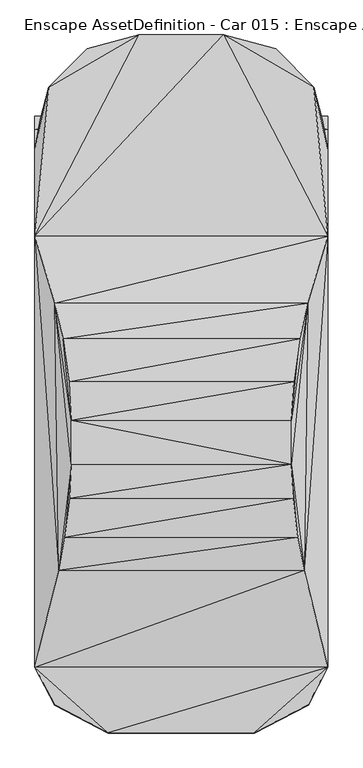
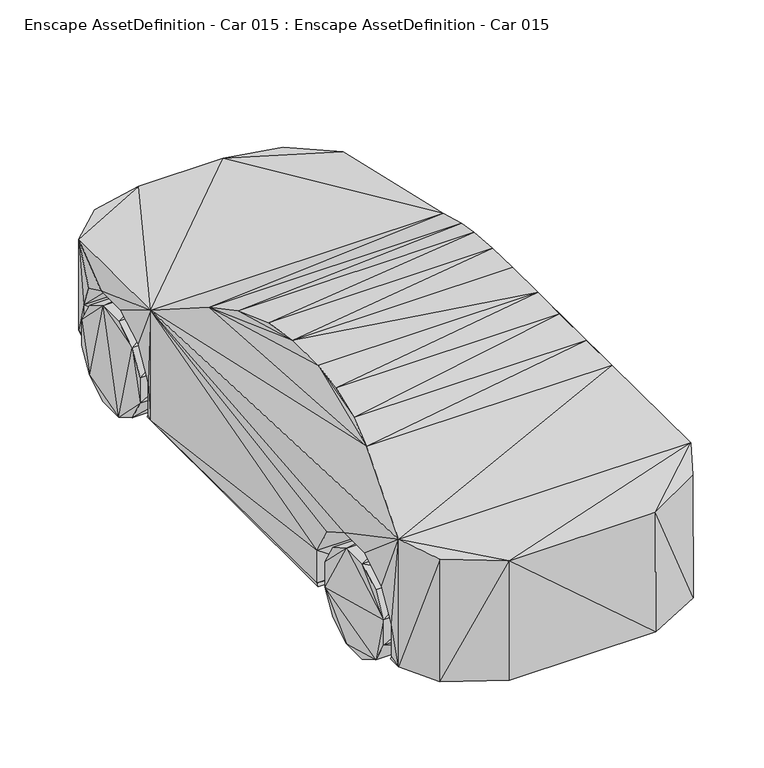
"""IFC4 building model written with IfcOpenShell, lengths in millimetres: geographic element geometry, Enscape AssetDefinition - Car 015 : Enscape AssetDefinition - Car 015."""

from ifc_helpers import new_model, si_unit, origin, place, context, project, spatial, faceted_brep, source, transform, mapped, element, save


def enscape_assetdefinition_car_015_enscape_assetdefinition_car_30b7849d(model_context):
    return source(origin(), model_context, "Body", "Brep", [
        faceted_brep([(944.226265, 1625.9566545, 237.0770574), (944.226265, 1386.8831396, 651.1646509), (944.226265, 1211.8692398, -1.9962895), (944.226265, 1538.4500027, 563.6575222), (641.0333514, 1538.4500027, 563.6575222), (641.033411, 1386.8831396, 651.1646509), (944.226265, 1211.8692398, 651.1646509), (944.226265, 1060.3027344, 563.6576414), (944.226265, 1625.9567738, 412.0909274), (944.226265, 972.7957845, 237.0771766), (641.0333514, 1625.9567738, 412.0909274), (641.0333514, 1625.9566545, 237.0770574), (641.033411, 1211.8692398, 651.1646509), (641.033411, 1060.3026152, 563.6576414), (944.226265, 972.7957845, 412.091136), (641.033411, 972.7957845, 412.091136), (641.0333514, 1211.8692398, -1.9962895), (641.0333514, 1538.449645, 85.5106041), (641.0333514, 972.7957845, 237.0771766), (944.226265, 1060.3026152, 85.5106935), (641.0333514, 1060.3026152, 85.5106935), (944.226265, 1386.8831396, -1.9963195), (944.226265, 1538.449645, 85.5105817), (641.0333514, 1386.8831396, -1.9963195)], [[[0, 1, 2]], [[3, 4, 1]], [[1, 5, 6]], [[7, 1, 6]], [[1, 0, 8]], [[1, 8, 3]], [[9, 1, 7]], [[1, 9, 2]], [[1, 4, 5]], [[10, 5, 4]], [[3, 10, 4]], [[8, 10, 3]], [[0, 11, 8]], [[8, 11, 10]], [[5, 10, 11]], [[11, 12, 5]], [[6, 5, 12]], [[6, 12, 7]], [[7, 13, 14]], [[9, 7, 14]], [[7, 12, 13]], [[15, 12, 11]], [[15, 13, 12]], [[16, 11, 17]], [[11, 16, 15]], [[0, 17, 11]], [[14, 15, 9]], [[16, 18, 15]], [[14, 13, 15]], [[9, 15, 18]], [[9, 18, 19]], [[18, 16, 20]], [[19, 18, 20]], [[19, 20, 2]], [[2, 9, 19]], [[2, 20, 16]], [[2, 16, 21]], [[22, 2, 21]], [[2, 22, 0]], [[22, 17, 0]], [[21, 23, 22]], [[22, 23, 17]], [[21, 16, 23]], [[16, 17, 23]]]),
        faceted_brep([(944.2260861, -1664.8235321, 85.5105221), (944.2260861, -1099.1698503, 237.0769083), (944.2261457, -1186.6767406, 563.657403), (944.2260861, -1186.6767406, 85.5104104), (641.0332918, -1186.6767406, 85.5104327), (944.2261457, -1099.1697311, 412.0908678), (641.0332918, -1099.1697311, 412.0908678), (944.2260861, -1338.2434845, -1.9965095), (641.0332918, -1099.1698503, 237.0769084), (641.0332918, -1338.2434845, -1.9965095), (944.2260861, -1513.2573843, -1.9964396), (641.0332918, -1513.2573843, -1.9964396), (641.0332918, -1664.8235321, 85.5105445), (641.0332918, -1186.6767406, 563.657403), (944.2261457, -1338.2434845, 651.1645317), (641.0332918, -1338.2434845, 651.1645317), (944.2261457, -1513.2570267, 651.1645317), (944.2260861, -1752.3306608, 237.0771319), (944.2260861, -1752.3306608, 412.090987), (641.0332322, -1752.3306608, 412.090987), (641.0332322, -1752.3306608, 237.0771319), (944.2261457, -1664.8238897, 563.6575818), (641.0332918, -1664.8238897, 563.6576414), (641.0332918, -1513.2570267, 651.1645317)], [[[0, 1, 2]], [[3, 4, 1]], [[5, 1, 6]], [[3, 1, 7]], [[1, 0, 7]], [[2, 1, 5]], [[1, 4, 8]], [[6, 1, 8]], [[9, 8, 4]], [[3, 9, 4]], [[7, 9, 3]], [[10, 11, 7]], [[7, 0, 10]], [[7, 11, 9]], [[11, 12, 9]], [[12, 8, 9]], [[12, 13, 8]], [[8, 13, 6]], [[2, 13, 14]], [[12, 15, 13]], [[2, 6, 13]], [[14, 13, 15]], [[14, 15, 16]], [[17, 14, 16]], [[14, 17, 0]], [[14, 0, 2]], [[5, 6, 2]], [[0, 12, 10]], [[0, 17, 12]], [[18, 19, 17]], [[18, 17, 16]], [[17, 19, 20]], [[12, 17, 20]], [[21, 22, 18]], [[18, 16, 21]], [[18, 22, 19]], [[21, 16, 22]], [[19, 22, 23]], [[22, 16, 23]], [[19, 23, 15]], [[16, 15, 23]], [[19, 15, 12]], [[19, 12, 20]], [[10, 12, 11]]]),
        faceted_brep([(-944.226265, 1060.3027344, 563.6576414), (-944.226265, 1211.8692398, -1.9962895), (-944.226265, 972.7957845, 237.0771766), (-944.226265, 1060.3026152, 85.5106935), (-641.0333514, 1060.3026152, 85.5106935), (-944.226265, 1386.8831396, -1.9963195), (-641.0333514, 1211.8692398, -1.9962895), (-944.226265, 1538.449645, 85.5105817), (-944.226265, 1386.8831396, 651.1646509), (-641.0333514, 972.7957845, 237.0771766), (-641.033411, 1386.8831396, 651.1646509), (-641.0333514, 1538.449645, 85.5106041), (-641.033411, 972.7957845, 412.091136), (-641.0333514, 1386.8831396, -1.9963195), (-944.226265, 1625.9566545, 237.0770574), (-641.0333514, 1625.9566545, 237.0770574), (-944.226265, 1625.9567738, 412.0909274), (-944.226265, 1538.4500027, 563.6575222), (-641.0333514, 1625.9567738, 412.0909274), (-641.0333514, 1538.4500027, 563.6575222), (-944.226265, 1211.8692398, 651.1646509), (-641.033411, 1211.8692398, 651.1646509), (-944.226265, 972.7957845, 412.091136), (-641.033411, 1060.3026152, 563.6576414)], [[[0, 1, 2]], [[3, 1, 4]], [[1, 5, 6]], [[1, 7, 5]], [[2, 1, 3]], [[1, 0, 8]], [[7, 1, 8]], [[4, 1, 6]], [[6, 9, 4]], [[9, 3, 4]], [[2, 3, 9]], [[10, 9, 11]], [[10, 12, 9]], [[11, 9, 6]], [[12, 2, 9]], [[11, 6, 13]], [[6, 5, 13]], [[5, 7, 13]], [[13, 7, 11]], [[7, 14, 11]], [[10, 11, 15]], [[11, 14, 15]], [[14, 16, 15]], [[7, 16, 14]], [[7, 8, 16]], [[16, 17, 18]], [[16, 8, 17]], [[15, 16, 18]], [[10, 15, 18]], [[10, 18, 19]], [[18, 17, 19]], [[17, 8, 19]], [[19, 8, 10]], [[8, 20, 10]], [[8, 0, 20]], [[20, 0, 21]], [[10, 20, 21]], [[0, 22, 23]], [[0, 2, 22]], [[21, 0, 23]], [[23, 10, 21]], [[10, 23, 12]], [[23, 22, 12]], [[22, 2, 12]]]),
        faceted_brep([(-944.2261457, -1338.2434845, 651.1645317), (-944.2260861, -1099.1698503, 237.0769083), (-944.2260861, -1752.3306608, 412.090987), (-944.2260861, -1186.6767406, 85.5104104), (-641.0332918, -1186.6767406, 85.5104327), (-641.0332918, -1099.1698503, 237.0769083), (-641.0332918, -1099.1697311, 412.0908678), (-944.2261457, -1099.1697311, 412.0908678), (-944.2260861, -1338.2434845, -1.9965095), (-944.2260861, -1664.8235321, 85.5105221), (-641.0332918, -1338.2434845, -1.9965095), (-944.2260861, -1513.2573843, -1.9964396), (-641.0332918, -1513.2573843, -1.9964396), (-641.0332918, -1664.8235321, 85.5105445), (-944.2260861, -1752.3306608, 237.0771319), (-641.0332918, -1338.2434845, 651.1645317), (-641.0332322, -1752.3306608, 237.0771319), (-641.0332322, -1752.3306608, 412.090987), (-944.2261457, -1664.8238897, 563.6575818), (-641.0332918, -1664.8238897, 563.6576414), (-944.2261457, -1513.2570267, 651.1645317), (-641.0332918, -1513.2570267, 651.1645317), (-641.0332918, -1186.6767406, 563.657403), (-944.2261457, -1186.6767406, 563.657403)], [[[0, 1, 2]], [[3, 1, 4]], [[5, 1, 6]], [[0, 7, 1]], [[8, 1, 3]], [[2, 1, 9]], [[9, 1, 8]], [[4, 1, 5]], [[6, 1, 7]], [[4, 5, 10]], [[10, 3, 4]], [[8, 3, 10]], [[11, 8, 12]], [[9, 8, 11]], [[12, 8, 10]], [[9, 11, 13]], [[2, 9, 14]], [[13, 14, 9]], [[13, 11, 12]], [[10, 13, 12]], [[5, 13, 10]], [[5, 15, 13]], [[16, 14, 13]], [[15, 16, 13]], [[2, 14, 17]], [[17, 14, 16]], [[18, 2, 19]], [[2, 18, 20]], [[2, 20, 0]], [[19, 2, 17]], [[17, 15, 21]], [[17, 21, 19]], [[15, 17, 16]], [[21, 20, 19]], [[19, 20, 18]], [[0, 20, 15]], [[15, 20, 21]], [[22, 15, 5]], [[22, 0, 15]], [[23, 0, 22]], [[7, 0, 23]], [[22, 5, 6]], [[6, 23, 22]], [[7, 23, 6]]]),
        faceted_brep([(-815.307498, 422.5830138, 1182.9679012), (-762.8209591, 193.0336207, 1280.1650763), (815.307498, 422.5830138, 1182.9679012), (-724.3981361, -82.6306492, 1351.3184786), (762.8209591, 193.0336207, 1280.1650763), (-710.3345394, -330.5457234, 1377.3621321), (724.3981361, -82.6306492, 1351.3184786), (710.3345394, -330.5457234, 1377.3621321), (710.3345394, -613.2781506, 1377.3621321), (-710.3345394, -613.2781506, 1377.3621321), (-721.2539911, -833.4584832, 1362.6734018), (751.0869503, -1083.989501, 1322.5426674), (791.8394208, -1297.7416515, 1267.7229643), (721.2539911, -833.4584832, 1362.6734018), (-791.8394208, -1297.7416515, 1267.7229643), (-751.0869503, -1083.989501, 1322.5426674), (-944.226265, -1921.1826324, 1062.7344847), (-944.226265, 854.2361856, 944.2293644), (944.226265, 854.2361856, 944.2293644), (944.226265, 1410.9764099, 741.0817742), (854.3379307, 1815.1055574, 814.7835732), (273.2906044, 2150.5734921, 769.5902586), (944.2261457, -1009.2525482, 436.1840785), (944.226265, 854.2361856, 194.9097514), (944.2261457, -1314.150095, 741.0815358), (944.226265, -1921.1826324, 1062.7344847), (944.2261457, -1120.8525896, 629.481256), (944.226265, 882.8786612, 436.1843765), (944.226265, 994.4790006, 629.481554), (944.226265, 1187.7760887, 741.081655), (617.3202395, -1009.2525482, 436.1840785), (617.3202395, -1120.8525896, 629.481256), (617.3202395, -1009.2526674, 212.9837573), (617.3202395, -1019.6877718, 194.9097514), (617.3202395, -1314.150095, 741.0815358), (944.2261457, -1537.350297, 741.0815358), (617.3202395, -1831.8123817, 194.9097514), (617.3202395, -1537.350297, 741.0815358), (944.2261457, -1730.6474447, 629.4814348), (617.3202395, -1730.6474447, 629.4814348), (944.226265, -1842.2478437, 436.1842871), (617.3202395, -1842.2478437, 436.1842871), (944.2261457, -1842.2474861, 212.9838914), (944.226265, -1921.1826324, 194.9097514), (617.3202395, -1842.2474861, 212.9838914), (944.226265, -1831.8123817, 194.9097514), (817.7238703, -2165.817976, 194.9097514), (817.7239299, -2163.7268066, 1030.8158398), (472.1131325, -2341.281414, 1007.4497461), (472.1130729, -2344.9032307, 194.9097514), (-472.1131325, -2341.281414, 1007.4497461), (-472.1130729, -2344.9032307, 194.9097514), (-617.3202395, -1831.8123817, 194.9097514), (-817.7238703, -2165.817976, 194.9097514), (-817.7239299, -2163.7268066, 1030.8158398), (-944.226265, -1921.1826324, 194.9097514), (-944.2261457, -1537.350297, 741.0815358), (-944.2261457, -1314.150095, 741.0815358), (-944.226265, -1842.2478437, 436.1842871), (-944.2261457, -1730.6474447, 629.4814348), (-944.226265, -1831.8123817, 194.9097514), (-944.2261457, -1842.2474861, 212.9838914), (-617.3202395, -1842.2478437, 436.1842871), (-617.3202395, -1537.350297, 741.0815358), (-617.3202395, -1730.6474447, 629.4814348), (-617.3202395, -1842.2474861, 212.9838914), (-617.3202395, -1019.6877718, 194.9097514), (-617.3202395, -1314.150095, 741.0815358), (-617.3202395, -1120.8525896, 629.481256), (-944.2261457, -1120.8525896, 629.481256), (-617.3202395, -1009.2525482, 436.1840785), (-944.2261457, -1009.2525482, 436.1840785), (-617.3202395, -1009.2526674, 212.9837573), (-944.2261457, -1009.2526674, 212.9837573), (-944.226265, 854.2361856, 194.9097514), (-944.226265, -1019.6877718, 194.9097514), (-595.2704549, 893.3138251, 194.9097514), (944.226265, -1019.6877718, 194.9097514), (944.2261457, -1009.2526674, 212.9837573), (595.2704549, 893.3138251, 194.9097514), (944.2261457, 893.3138251, 194.9097514), (944.226265, 882.8786612, 212.9839808), (595.2704549, 882.8786612, 212.9839808), (595.2704549, 882.8786612, 436.1843765), (595.2704549, 994.4790006, 629.481554), (595.2704549, 1187.7760887, 741.081655), (595.2704549, 1410.9764099, 741.0817742), (595.2704549, 1705.4384947, 194.9097514), (595.2704549, 1604.2739153, 629.4813752), (910.8301997, 1604.2739153, 629.4813752), (880.9269071, 1715.8739567, 436.1840785), (595.2704549, 1715.8739567, 436.1840785), (880.9269667, 1715.8735991, 212.9838467), (595.2704549, 1715.8735991, 212.9838467), (854.3379903, 1815.1054382, 194.9097514), (608.7583899, 2060.6849194, 781.6997766), (608.7583899, 2060.6849194, 194.9097514), (883.7230802, 1705.4384947, 194.9097514), (-595.2704549, 1705.4384947, 194.9097514), (-273.2906044, 2150.5734921, 194.9097514), (273.2906044, 2150.5734921, 194.9097514), (-273.2906044, 2150.5734921, 769.5902586), (-608.7583899, 2060.6849194, 194.9097514), (-854.3379307, 1815.1055574, 814.7835732), (-608.7583899, 2060.6849194, 781.6997766), (-854.3379903, 1815.1054382, 194.9097514), (-944.226265, 1410.9764099, 741.0817742), (-880.9269071, 1715.8739567, 436.1840785), (-910.8301997, 1604.2739153, 629.4813752), (-883.7230802, 1705.4384947, 194.9097514), (-880.9269667, 1715.8735991, 212.9838467), (-595.2704549, 1715.8735991, 212.9838467), (-595.2704549, 1604.2739153, 629.4813752), (-595.2704549, 1715.8739567, 436.1840785), (-595.2704549, 1410.9764099, 741.0817742), (-595.2704549, 1187.7760887, 741.081655), (-944.226265, 1187.7760887, 741.081655), (-944.226265, 994.4790006, 629.481554), (-595.2704549, 994.4790006, 629.481554), (-944.226265, 882.8786612, 436.1843765), (-595.2704549, 882.8786612, 436.1843765), (-944.226265, 882.8786612, 212.9839808), (-595.2704549, 882.8786612, 212.9839808), (-944.2261457, 893.3138251, 194.9097514)], [[[0, 1, 2]], [[1, 3, 4]], [[2, 1, 4]], [[1, 5, 3]], [[5, 1, 0]], [[3, 5, 6]], [[4, 3, 6]], [[7, 2, 4]], [[7, 4, 6]], [[6, 5, 7]], [[7, 5, 8]], [[8, 5, 9]], [[0, 9, 5]], [[2, 7, 8]], [[9, 10, 8]], [[8, 11, 12]], [[8, 10, 13]], [[8, 12, 2]], [[11, 8, 13]], [[9, 0, 14]], [[9, 14, 15]], [[9, 15, 10]], [[10, 15, 13]], [[13, 15, 11]], [[15, 14, 11]], [[11, 14, 12]], [[14, 16, 12]], [[14, 17, 16]], [[14, 0, 17]], [[17, 0, 18]], [[18, 0, 2]], [[12, 18, 2]], [[18, 19, 20]], [[21, 17, 18]], [[21, 18, 20]], [[22, 23, 18]], [[24, 18, 25]], [[18, 26, 22]], [[18, 24, 26]], [[18, 12, 25]], [[27, 18, 23]], [[28, 18, 27]], [[29, 18, 28]], [[18, 29, 19]], [[22, 26, 30]], [[26, 24, 31]], [[30, 26, 31]], [[32, 22, 30]], [[30, 33, 32]], [[30, 31, 33]], [[31, 24, 34]], [[33, 31, 34]], [[24, 35, 34]], [[36, 34, 37]], [[34, 35, 37]], [[34, 36, 33]], [[25, 35, 24]], [[35, 38, 37]], [[35, 25, 38]], [[37, 38, 39]], [[36, 37, 39]], [[38, 40, 39]], [[38, 25, 40]], [[39, 40, 41]], [[36, 39, 41]], [[40, 42, 41]], [[40, 43, 42]], [[40, 25, 43]], [[41, 42, 44]], [[36, 41, 44]], [[44, 42, 36]], [[42, 43, 45]], [[36, 42, 45]], [[46, 43, 47]], [[43, 36, 45]], [[36, 43, 46]], [[47, 43, 25]], [[48, 46, 47]], [[48, 47, 25]], [[49, 46, 48]], [[36, 46, 49]], [[25, 50, 48]], [[50, 49, 48]], [[51, 49, 50]], [[36, 49, 51]], [[36, 51, 52]], [[52, 33, 36]], [[52, 51, 53]], [[50, 53, 51]], [[54, 53, 50]], [[50, 25, 16]], [[50, 16, 54]], [[12, 16, 25]], [[16, 55, 54]], [[56, 16, 57]], [[57, 16, 17]], [[16, 58, 55]], [[16, 59, 58]], [[16, 56, 59]], [[54, 55, 53]], [[52, 53, 55]], [[52, 55, 60]], [[55, 61, 60]], [[55, 58, 61]], [[58, 62, 61]], [[58, 59, 62]], [[56, 63, 59]], [[59, 63, 64]], [[62, 59, 64]], [[62, 52, 65]], [[61, 62, 65]], [[52, 62, 64]], [[60, 61, 52]], [[52, 61, 65]], [[66, 33, 52]], [[52, 64, 63]], [[52, 63, 67]], [[67, 66, 52]], [[56, 67, 63]], [[57, 67, 56]], [[57, 68, 67]], [[66, 67, 68]], [[69, 68, 57]], [[69, 57, 17]], [[69, 70, 68]], [[66, 68, 70]], [[71, 70, 69]], [[17, 71, 69]], [[71, 72, 70]], [[66, 70, 72]], [[73, 72, 71]], [[71, 17, 74]], [[71, 74, 73]], [[73, 66, 72]], [[75, 66, 73]], [[73, 74, 75]], [[74, 66, 75]], [[76, 33, 66]], [[76, 66, 74]], [[77, 78, 33]], [[33, 23, 77]], [[79, 23, 33]], [[79, 33, 76]], [[33, 78, 32]], [[78, 22, 32]], [[23, 78, 77]], [[23, 22, 78]], [[79, 80, 23]], [[81, 23, 80]], [[27, 23, 81]], [[81, 80, 82]], [[82, 80, 79]], [[27, 81, 83]], [[83, 81, 82]], [[28, 27, 84]], [[84, 27, 83]], [[79, 84, 83]], [[79, 83, 82]], [[85, 28, 84]], [[79, 85, 84]], [[29, 28, 85]], [[86, 29, 85]], [[87, 86, 85]], [[85, 79, 87]], [[19, 29, 86]], [[88, 89, 86]], [[86, 89, 19]], [[87, 88, 86]], [[20, 19, 89]], [[20, 89, 90]], [[88, 90, 89]], [[91, 90, 88]], [[91, 88, 87]], [[92, 90, 93]], [[90, 92, 94]], [[90, 94, 20]], [[93, 90, 91]], [[20, 94, 95]], [[21, 20, 95]], [[87, 96, 94]], [[87, 94, 97]], [[95, 94, 96]], [[94, 92, 97]], [[97, 92, 87]], [[87, 92, 93]], [[91, 87, 93]], [[87, 98, 99]], [[87, 99, 100]], [[87, 100, 96]], [[98, 87, 79]], [[95, 96, 21]], [[21, 96, 100]], [[21, 101, 17]], [[100, 101, 21]], [[99, 101, 100]], [[99, 98, 102]], [[102, 101, 99]], [[103, 101, 104]], [[104, 101, 102]], [[101, 103, 17]], [[102, 98, 105]], [[105, 104, 102]], [[103, 104, 105]], [[103, 106, 17]], [[107, 103, 105]], [[108, 103, 107]], [[106, 103, 108]], [[105, 98, 109]], [[110, 105, 109]], [[107, 105, 110]], [[109, 98, 110]], [[110, 111, 107]], [[110, 98, 111]], [[108, 107, 112]], [[112, 107, 113]], [[107, 111, 113]], [[106, 108, 114]], [[114, 108, 112]], [[98, 114, 112]], [[98, 112, 113]], [[98, 113, 111]], [[79, 76, 98]], [[98, 115, 114]], [[115, 98, 76]], [[106, 114, 116]], [[116, 114, 115]], [[116, 115, 117]], [[76, 118, 115]], [[117, 115, 118]], [[17, 116, 117]], [[17, 106, 116]], [[117, 118, 119]], [[17, 117, 119]], [[119, 118, 120]], [[76, 120, 118]], [[119, 120, 121]], [[119, 121, 74]], [[119, 74, 17]], [[121, 120, 122]], [[120, 76, 122]], [[121, 122, 123]], [[74, 121, 123]], [[76, 74, 123]], [[123, 122, 76]]]),
    ])


if __name__ == "__main__":
    model = new_model("IFC4")
    model_context = context("Model", 3, world=origin())
    ifc_project = project(units=[si_unit("LENGTHUNIT", "METRE", prefix="MILLI")], contexts=[model_context])
    site = spatial("IfcSite", under=ifc_project)
    building = spatial("IfcBuilding", under=site)
    placement = place(None, origin())
    enscape_assetdefinition_car_015_enscape_assetdefinition_car_shape = enscape_assetdefinition_car_015_enscape_assetdefinition_car_30b7849d(model_context)
    element("IfcGeographicElement", 1, ObjectType="Enscape AssetDefinition - Car 015 : Enscape AssetDefinition - Car 015", at=placement, inside=building, context=model_context, shape_type="MappedRepresentation", body=[
        mapped(enscape_assetdefinition_car_015_enscape_assetdefinition_car_shape, transform((0.0, 0.0, 0.0), x_axis=(1.0, 0.0, 0.0), y_axis=(0.0, 1.0, 0.0), z_axis=(0.0, 0.0, 1.0))),
    ])
    save(model, "model.ifc")

# Revit data of these elements
# Type "Enscape AssetDefinition - Car 015 : Enscape AssetDefinition - Car 015"
#   EnscapeAssetSource = "REMOTE"
#   EnscapeAssetId = "90b8357f-f38c-4bd4-beff-0116ac26bef3"
#   Height = 1377.362 mm
#   EnscapeNativeAssetHeight = 1377.362 mm
#   Default Elevation = 0
